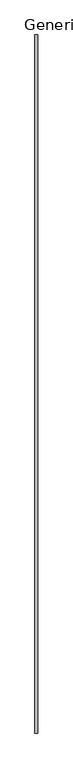
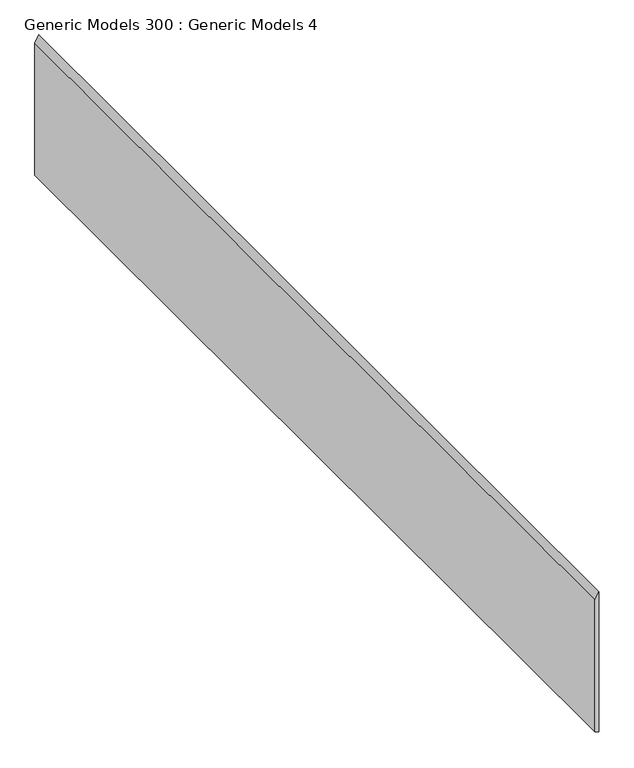
"""IFC4 building model written with IfcOpenShell, lengths in millimetres: proxy geometry, Generic Models 300 : Generic Models 4."""

from ifc_helpers import new_model, si_unit, frame, origin, place, context, project, spatial, polyline, outline, extrude, source, transform, mapped, element, save


def generic_models_300_generic_models_4_bd9cd6b2(model_context):
    return source(origin(), model_context, "Body", "SweptSolid", [
        extrude(outline(polyline([(124149.4118493, 6876.7852461), (123441.2995045, 6876.7852461), (123435.1470003, 6895.9263704), (124186.6866705, 6895.9263704), (124149.4118493, 6876.7852461)])), frame((0.0, 6851.0769662, 0.0), z_axis=(0.0, 1.0, 0.0), x_axis=(0.0, 0.0, 1.0)), (0.0, 0.0, 1.0), 4927.6),
    ])


if __name__ == "__main__":
    model = new_model("IFC4")
    model_context = context("Model", 3, world=origin())
    ifc_project = project(units=[si_unit("LENGTHUNIT", "METRE", prefix="MILLI")], contexts=[model_context])
    site = spatial("IfcSite", under=ifc_project)
    building = spatial("IfcBuilding", under=site)
    placement = place(None, origin())
    generic_models_300_generic_models_4_shape = generic_models_300_generic_models_4_bd9cd6b2(model_context)
    element("IfcBuildingElementProxy", 1, Name="Generic Models 300 : Generic Models 4", ObjectType="Generic Models 300 : Generic Models 4", at=placement, inside=building, context=model_context, shape_type="MappedRepresentation", body=[
        mapped(generic_models_300_generic_models_4_shape, transform((0.0, 0.0, 0.0), x_axis=(1.0, 0.0, 0.0), y_axis=(0.0, 1.0, 0.0), z_axis=(0.0, 0.0, 1.0))),
    ])
    save(model, "model.ifc")

# Revit data of these elements
# Element 1 (IfcBuildingElementProxy, "Generic Models 300 : Generic Models 4")
#   Materials on its faces: "_7/8\" SMOOTH TROWEL EXTERIOR STUCCO (COLOR PER OWNER)"
# Materials
#   "_7/8\" SMOOTH TROWEL EXTERIOR STUCCO (COLOR PER OWNER)": class "Generic", colour RGB 233 233 233, transparency 0, Cost = 0
